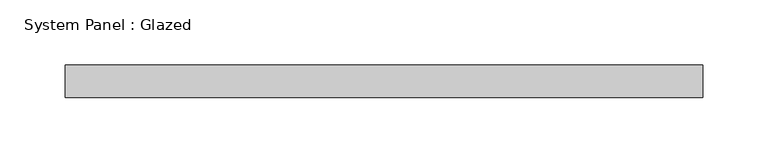
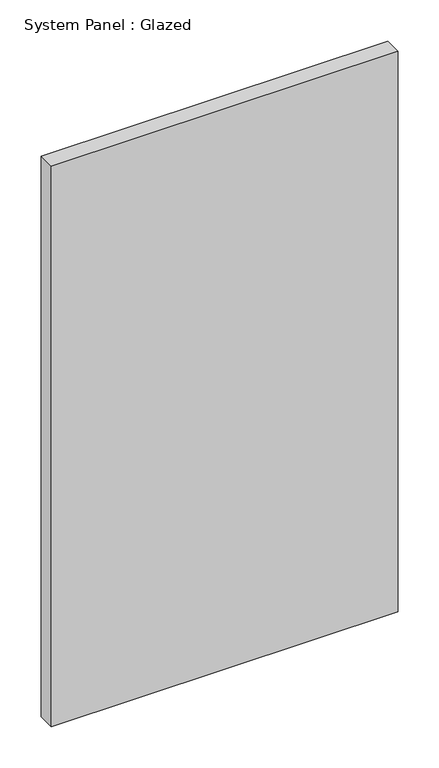
"""IFC4 building model written with IfcOpenShell, lengths in millimetres: plate geometry, System Panel : Glazed."""

from ifc_helpers import new_model, si_unit, origin, origin_with_axes, place, context, project, spatial, polyline, outline, extrude, source, transform, mapped, element, save


def system_panel_glazed_8e5c0314(model_context):
    return source(origin(), model_context, "Body", "SweptSolid", [
        extrude(outline(polyline([(243.9393939, 24.5), (-243.9393939, 24.5), (-243.9393939, 49.5), (243.9393939, 49.5), (243.9393939, 24.5)])), origin_with_axes(), (0.0, 0.0, 1.0), 833.3333333),
    ])


if __name__ == "__main__":
    model = new_model("IFC4")
    model_context = context("Model", 3, world=origin())
    ifc_project = project(units=[si_unit("LENGTHUNIT", "METRE", prefix="MILLI")], contexts=[model_context])
    site = spatial("IfcSite", under=ifc_project)
    building = spatial("IfcBuilding", under=site)
    placement = place(None, origin())
    system_panel_glazed_shape = system_panel_glazed_8e5c0314(model_context)
    element("IfcPlate", 1, ObjectType="System Panel : Glazed", at=placement, inside=building, context=model_context, shape_type="MappedRepresentation", body=[
        mapped(system_panel_glazed_shape, transform((0.0, 0.0, 0.0), x_axis=(1.0, 0.0, 0.0), y_axis=(0.0, 1.0, 0.0), z_axis=(0.0, 0.0, 1.0))),
    ])
    save(model, "model.ifc")

# Revit data of these elements
# Element 1 (IfcPlate, "System Panel : Glazed")
#   Materials on its faces: "Glass"
# Materials
#   "Glass": class "Glass", colour RGB 218 227 224, transparency 0.85, Description = "Soda Lime Glass", Cost = 0
